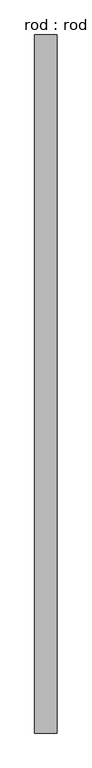
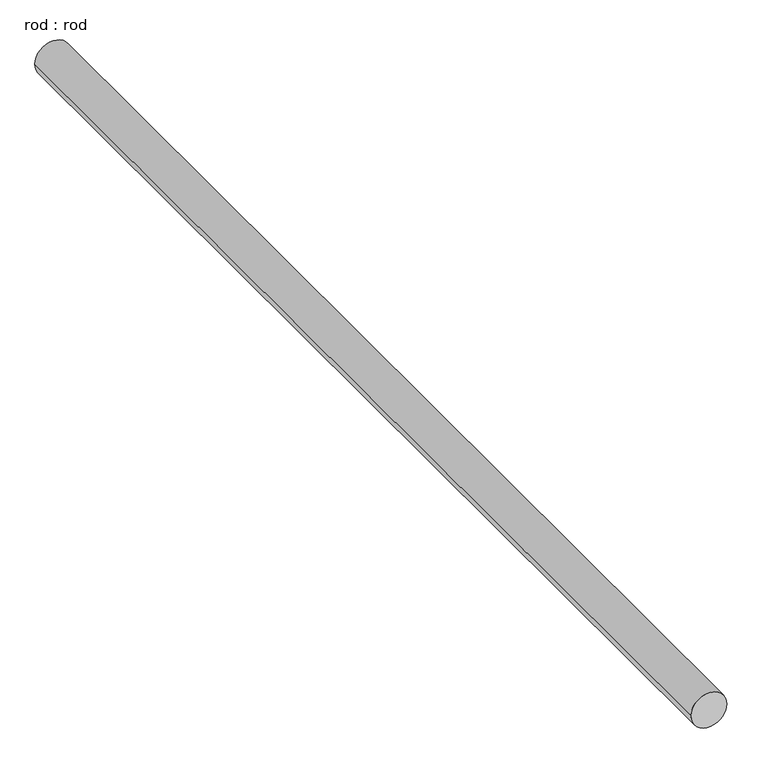
"""IFC4 building model written with IfcOpenShell, lengths in millimetres: proxy geometry, rod : rod."""

from ifc_helpers import new_model, si_unit, point, frame, frame_2d, origin, place, context, project, spatial, circle_curve, trimmed, segment, composite_curve, outline, extrude, source, transform, mapped, element, save


def rod_rod_37ee2bfa(model_context):
    return source(origin(), model_context, "Body", "SweptSolid", [
        extrude(outline(composite_curve([segment(trimmed(circle_curve(frame_2d((0.0108462, 0.0)), 200.0), [point((0.0108462, 200.0))], [point((0.0108462, -200.0))], False, "CARTESIAN"), True, "CONTINUOUS"), segment(trimmed(circle_curve(frame_2d((0.0108462, 0.0)), 200.0), [point((0.0108462, -200.0))], [point((0.0108462, 200.0))], False, "CARTESIAN"), True, "CONTINUOUS")], self_intersect=False)), frame((0.0, -2187.6551558, 0.0), z_axis=(0.0, 1.0, 0.0), x_axis=(0.0, 0.0, 1.0)), (0.0, 0.0, 1.0), 12560.7675422),
    ])


if __name__ == "__main__":
    model = new_model("IFC4")
    model_context = context("Model", 3, world=origin())
    ifc_project = project(units=[si_unit("LENGTHUNIT", "METRE", prefix="MILLI")], contexts=[model_context])
    site = spatial("IfcSite", under=ifc_project)
    building = spatial("IfcBuilding", under=site)
    placement = place(None, origin())
    rod_rod_shape = rod_rod_37ee2bfa(model_context)
    element("IfcBuildingElementProxy", 1, Name="rod : rod", ObjectType="rod : rod", at=placement, inside=building, context=model_context, shape_type="MappedRepresentation", body=[
        mapped(rod_rod_shape, transform((0.0, 0.0, 0.0), x_axis=(1.0, 0.0, 0.0), y_axis=(0.0, 1.0, 0.0), z_axis=(0.0, 0.0, 1.0))),
    ])
    save(model, "model.ifc")

# Revit data of these elements
# Type "rod : rod"
#   Default Elevation = 0
